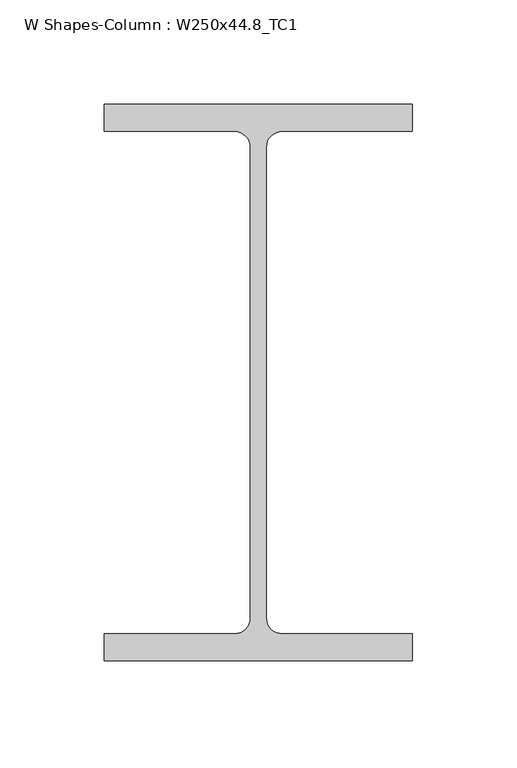
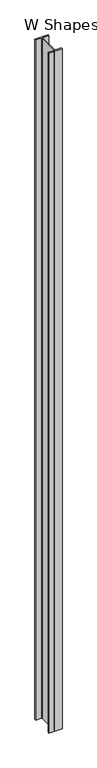
"""IFC4 building model written with IfcOpenShell, lengths in millimetres: column geometry, W Shapes-Column : W250x44.8_TC1."""

from ifc_helpers import new_model, si_unit, point, frame, frame_2d, origin, place, context, project, spatial, polyline, circle_curve, trimmed, segment, composite_curve, outline, extrude, source, transform, mapped, element, save


def w_shapes_column_w250x44_8_tc1_9eb3ea08(model_context):
    return source(origin(), model_context, "Body", "SweptSolid", [
        extrude(outline(composite_curve([segment(polyline([(73.787, -133.35), (-73.787, -133.35), (-73.787, -120.396), (-11.43, -120.396)]), True, "CONTINUOUS"), segment(trimmed(circle_curve(frame_2d((-11.43, -112.776)), 7.62), [point((-11.43, -120.396))], [point((-3.81, -112.776))], True, "CARTESIAN"), True, "CONTINUOUS"), segment(polyline([(-3.81, -112.776), (-3.81, 112.776)]), True, "CONTINUOUS"), segment(trimmed(circle_curve(frame_2d((-11.43, 112.776)), 7.62), [point((-3.81, 112.776))], [point((-11.43, 120.396))], True, "CARTESIAN"), True, "CONTINUOUS"), segment(polyline([(-11.43, 120.396), (-73.787, 120.396), (-73.787, 133.35), (73.787, 133.35), (73.787, 120.396), (11.43, 120.396)]), True, "CONTINUOUS"), segment(trimmed(circle_curve(frame_2d((11.43, 112.776)), 7.62), [point((11.43, 120.396))], [point((3.81, 112.776))], True, "CARTESIAN"), True, "CONTINUOUS"), segment(polyline([(3.81, 112.776), (3.81, -112.776)]), True, "CONTINUOUS"), segment(trimmed(circle_curve(frame_2d((11.43, -112.776)), 7.62), [point((3.81, -112.776))], [point((11.43, -120.396))], True, "CARTESIAN"), True, "CONTINUOUS"), segment(polyline([(11.43, -120.396), (73.787, -120.396), (73.787, -133.35)]), True, "CONTINUOUS")], self_intersect=False)), frame((0.0, 0.0, 200.0), z_axis=(0.0, 0.0, 1.0), x_axis=(1.0, 0.0, 0.0)), (0.0, 0.0, 1.0), 8000.0),
    ])


if __name__ == "__main__":
    model = new_model("IFC4")
    model_context = context("Model", 3, world=origin())
    ifc_project = project(units=[si_unit("LENGTHUNIT", "METRE", prefix="MILLI")], contexts=[model_context])
    site = spatial("IfcSite", under=ifc_project)
    building = spatial("IfcBuilding", under=site)
    placement = place(None, origin())
    w_shapes_column_w250x44_8_tc1_shape = w_shapes_column_w250x44_8_tc1_9eb3ea08(model_context)
    element("IfcColumn", 1, ObjectType="W Shapes-Column : W250x44.8_TC1", at=placement, inside=building, context=model_context, shape_type="MappedRepresentation", body=[
        mapped(w_shapes_column_w250x44_8_tc1_shape, transform((0.0, 0.0, 0.0), x_axis=(1.0, 0.0, 0.0), y_axis=(0.0, 1.0, 0.0), z_axis=(0.0, 0.0, 1.0))),
    ])
    save(model, "model.ifc")

# Revit data of these elements
# Type "W Shapes-Column : W250x44.8_TC1"
#   Section Name Key = "W10X30"
#   Assembly Code = "B10"
#   Width = 14.7574 cm
#   Web Thickness = 0.762 cm
#   Web Fillet = 0.762 cm
#   Warping Constant = 111173.8 cm⁶
#   Torsional Moment of Inertia = 25.8896 cm⁴
#   Section Area = 57.0321 cm²
#   Plastic Modulus weak axis = 144.862 cm³
#   Plastic Modulus strong axis = 599.767 cm³
#   Perimeter = 1.09454 m²/m
#   Nominal Weight = 44.6449 kgf/m
#   Moment of Inertia weak axis = 695.106 cm⁴
#   Moment of Inertia strong axis = 7075.93 cm⁴
#   Height = 26.67 cm
#   Flange Thickness = 1.2954 cm
#   Elastic Modulus weak axis = 94.2256 cm³
#   Elastic Modulus strong axis = 530.941 cm³
#   Clear Web Height = 20.955 cm
#   Centroid Vertical = 13.335 cm
#   Centroid Horizontal = 7.3787 cm
#   Bolt Spacing = 6.985 cm
#   Structural Material [instance default] = Steel ASTM A992
#   Principal Axes Angle = 0
# Element 1 (IfcColumn, "W Shapes-Column : W250x44.8_TC1")
#   Structural Material = none
# Materials
#   "Steel ASTM A992": class "Metal", colour RGB 199 199 199, transparency 0, Description = "Structural steel 50ksi", Cost = 0
